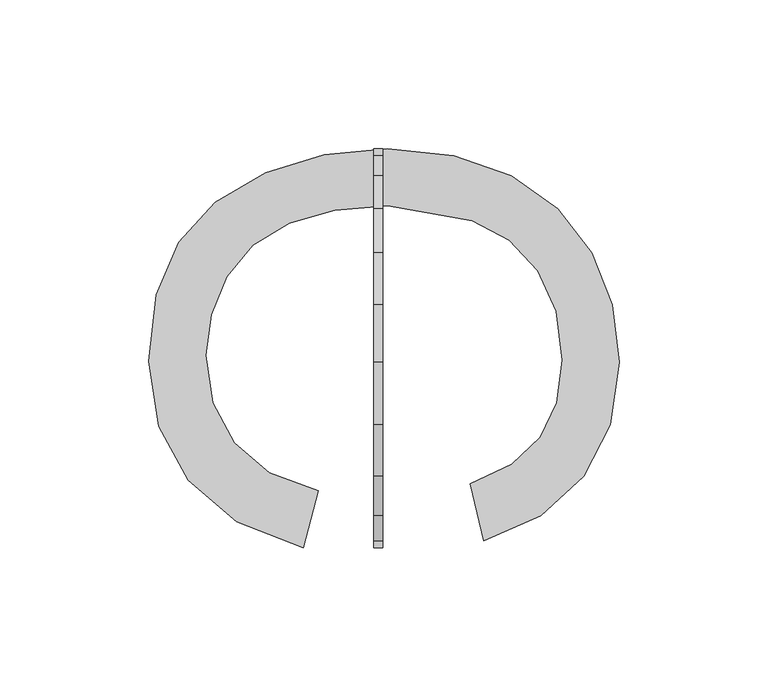
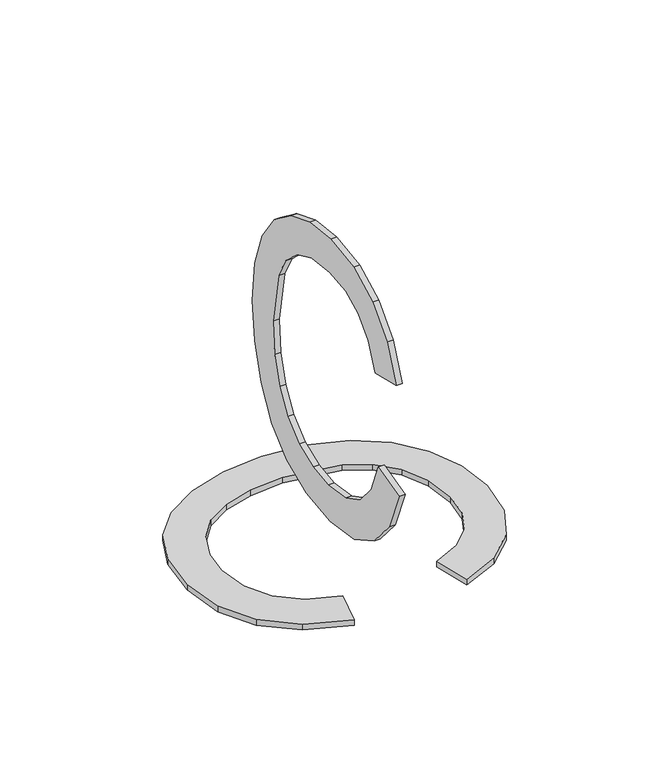
"""IFC4 building model written with IfcOpenShell, lengths in millimetres: proxy geometry, Grid Number2_FedEx : Grid Number2_FedEx."""

import ifcopenshell
import ifcopenshell.guid

model = None  # the IFC model being written
_history = None  # IfcOwnerHistory: only IFC2X3 demands one
_inside = {}  # id of a spatial element -> (the spatial element, [elements in it])
_under = {}  # id of a project, library or spatial element -> (it, [spatial elements below it])
_declared = {}  # id of a project -> (the project, [libraries it declares])
_typed = {}  # id of a type object -> (the type object, [elements of that type])
_made_of = {}  # id of a material, layer set ... -> (it, [elements and type objects made of it])


def new_model(schema):
    """Start an empty IFC model of exactly this schema.

    Asked for "IFC4X3", IfcOpenShell would pick the latest addendum, in which some entities
    have other attributes; the version numbers below select the first issue.
    IFC2X3 requires an IfcOwnerHistory on every rooted entity: one is made here for all.
    """
    global model, _history
    if schema == "IFC4X3":
        model = ifcopenshell.file(schema_version=(4, 3, 0, 0))
    else:
        model = ifcopenshell.file(schema=schema)
    _inside.clear()
    _under.clear()
    _declared.clear()
    _typed.clear()
    _made_of.clear()
    _history = None
    if model.schema == "IFC2X3":
        org = make("IfcOrganization", Name="unknown")
        user = make(
            "IfcPersonAndOrganization",
            ThePerson=make("IfcPerson", FamilyName="unknown"),
            TheOrganization=org,
        )
        app = make(
            "IfcApplication",
            ApplicationDeveloper=org,
            Version="unknown",
            ApplicationFullName="unknown",
            ApplicationIdentifier="unknown",
        )
        _history = make(
            "IfcOwnerHistory",
            OwningUser=user,
            OwningApplication=app,
            ChangeAction="ADDED",
            CreationDate=0,
        )
    return model


def make(cls, **values):
    """One entity of the class cls with the attributes given. An attribute that is None is left unset."""
    return model.create_entity(
        cls, **{name: value for name, value in values.items() if value is not None}
    )


def rooted(cls, **values):
    """An entity with a GlobalId (a new one), such as an element, a storey or a relation."""
    return make(cls, GlobalId=ifcopenshell.guid.new(), OwnerHistory=_history, **values)


def si_unit(unit_type, name, prefix=None):
    """IfcSIUnit, for example si_unit("LENGTHUNIT", "METRE", prefix="MILLI")."""
    return make("IfcSIUnit", UnitType=unit_type, Prefix=prefix, Name=name)


def assignment(units):
    """IfcUnitAssignment: the units of a project."""
    return None if units is None else make("IfcUnitAssignment", Units=units)


def point(xyz):
    """IfcCartesianPoint."""
    return None if xyz is None else make("IfcCartesianPoint", Coordinates=xyz)


def direction(xyz):
    """IfcDirection."""
    return None if xyz is None else make("IfcDirection", DirectionRatios=xyz)


def frame(location, z_axis=None, x_axis=None):
    """IfcAxis2Placement3D, a coordinate frame: its origin and axes. An axis left out is left unset."""
    return make(
        "IfcAxis2Placement3D",
        Location=point(location),
        Axis=direction(z_axis),
        RefDirection=direction(x_axis),
    )


def origin():
    """The frame at (0, 0, 0) with its axes left unset."""
    return frame((0.0, 0.0, 0.0))


def origin_with_axes():
    """The frame at (0, 0, 0) with the z axis (0, 0, 1) and the x axis (1, 0, 0) written out."""
    return frame((0.0, 0.0, 0.0), z_axis=(0.0, 0.0, 1.0), x_axis=(1.0, 0.0, 0.0))


def place(relative_to, where):
    """IfcLocalPlacement: puts the frame where relative to a parent placement (None: the world)."""
    return make(
        "IfcLocalPlacement", PlacementRelTo=relative_to, RelativePlacement=where
    )


def context(
    kind, dimensions, precision=None, world=None, true_north=None, identifier=None
):
    """IfcGeometricRepresentationContext, for example the 3D "Model" context."""
    return make(
        "IfcGeometricRepresentationContext",
        ContextIdentifier=identifier,
        ContextType=kind,
        CoordinateSpaceDimension=dimensions,
        Precision=precision,
        WorldCoordinateSystem=world,
        TrueNorth=true_north,
    )


def project(units=None, contexts=None):
    """IfcProject with its units and contexts."""
    return rooted(
        "IfcProject",
        Name="project",
        RepresentationContexts=contexts,
        UnitsInContext=assignment(units),
    )


def spatial(cls, under=None, at=None, **own):
    """A site, building, storey or space (cls), placed at a placement, below another one or the project."""
    s = rooted(cls, ObjectPlacement=at, **own)
    if under is not None:
        _under.setdefault(under.id(), (under, []))[1].append(s)
    return s


def polyline(points):
    """IfcPolyline through the points."""
    return make("IfcPolyline", Points=[point(p) for p in points])


def outline(outer, holes=None, kind="AREA"):
    """IfcArbitraryClosedProfileDef: a profile drawn as a closed curve; with holes, ...WithVoids."""
    if holes is None:
        return make("IfcArbitraryClosedProfileDef", ProfileType=kind, OuterCurve=outer)
    return make(
        "IfcArbitraryProfileDefWithVoids",
        ProfileType=kind,
        OuterCurve=outer,
        InnerCurves=holes,
    )


def extrude(swept, where, along, depth):
    """IfcExtrudedAreaSolid: the profile swept, set in the frame where, extruded along a direction by depth."""
    return make(
        "IfcExtrudedAreaSolid",
        SweptArea=swept,
        Position=where,
        ExtrudedDirection=direction(along),
        Depth=depth,
    )


def shape(context_of_items, identifier, shape_type, items):
    """IfcShapeRepresentation: the items that make up one representation, for example the "Body"."""
    return make(
        "IfcShapeRepresentation",
        ContextOfItems=context_of_items,
        RepresentationIdentifier=identifier,
        RepresentationType=shape_type,
        Items=items,
    )


def source(mapping_origin, context_of_items, identifier, shape_type, items):
    """IfcRepresentationMap: a shape defined once, which mapped items show again and again."""
    return make(
        "IfcRepresentationMap",
        MappingOrigin=mapping_origin,
        MappedRepresentation=shape(context_of_items, identifier, shape_type, items),
    )


def transform(
    local_origin,
    x_axis=None,
    y_axis=None,
    z_axis=None,
    scale=None,
    scale2=None,
    scale3=None,
    uniform=True,
):
    """IfcCartesianTransformationOperator3D, or its non-uniform kind. x_axis, y_axis, z_axis: its Axis1, 2, 3."""
    if uniform:
        return make(
            "IfcCartesianTransformationOperator3D",
            Axis1=direction(x_axis),
            Axis2=direction(y_axis),
            LocalOrigin=point(local_origin),
            Scale=scale,
            Axis3=direction(z_axis),
        )
    return make(
        "IfcCartesianTransformationOperator3DnonUniform",
        Axis1=direction(x_axis),
        Axis2=direction(y_axis),
        LocalOrigin=point(local_origin),
        Scale=scale,
        Axis3=direction(z_axis),
        Scale2=scale2,
        Scale3=scale3,
    )


def mapped(mapping_source, mapping_target):
    """IfcMappedItem: shows the shape of a source again, moved by a transform."""
    return make(
        "IfcMappedItem", MappingSource=mapping_source, MappingTarget=mapping_target
    )


def made_of(thing, what):
    """Note that an element or type object is made of a material, layer set ...; save() writes the relation."""
    if what is not None:
        _made_of.setdefault(what.id(), (what, []))[1].append(thing)
    return thing


def element(
    cls,
    number,
    at=None,
    inside=None,
    cuts=None,
    type_object=None,
    material=None,
    context=None,
    identifier="Body",
    shape_type=None,
    held_by="IfcProductDefinitionShape",
    body=None,
    shapes=None,
    **own,
):
    """One element of the class cls, such as IfcWall. Its Tag is "e" and its number.

    at: its placement. inside: the storey or other place that contains it. cuts: it is an
    opening in that element (IfcRelVoidsElement). A single representation is given by context,
    identifier, shape_type and body (its items); several are given by shapes. held_by: the class
    of the entity that holds the representations. save() writes the other relations.
    """
    e = rooted(cls, Tag="e%d" % number, ObjectPlacement=at, **own)
    if body is not None:
        shapes = [shape(context, identifier, shape_type, body)]
    if shapes is not None:
        e.Representation = make(held_by, Representations=shapes)
    if inside is not None:
        _inside.setdefault(inside.id(), (inside, []))[1].append(e)
    if cuts is not None:
        rooted(
            "IfcRelVoidsElement", RelatingBuildingElement=cuts, RelatedOpeningElement=e
        )
    if type_object is not None:
        _typed.setdefault(type_object.id(), (type_object, []))[1].append(e)
    return made_of(e, material)


def aggregate(whole, parts):
    """IfcRelAggregates: a whole, such as a stair, and the parts it consists of."""
    return rooted("IfcRelAggregates", RelatingObject=whole, RelatedObjects=parts)


def save(model, path):
    """Write the relations noted so far, then the file.

    IfcRelAggregates (storeys below a building ...), IfcRelContainedInSpatialStructure (elements
    in a storey), IfcRelDefinesByType, IfcRelAssociatesMaterial and IfcRelDeclares: one each for
    every whole, place, type object, material and project.
    """
    for whole, parts in _under.values():
        aggregate(whole, parts)
    for where, things in _inside.values():
        rooted(
            "IfcRelContainedInSpatialStructure",
            RelatedElements=things,
            RelatingStructure=where,
        )
    for kind, things in _typed.values():
        rooted("IfcRelDefinesByType", RelatedObjects=things, RelatingType=kind)
    for what, things in _made_of.values():
        rooted("IfcRelAssociatesMaterial", RelatedObjects=things, RelatingMaterial=what)
    for by, libraries in _declared.values():
        rooted("IfcRelDeclares", RelatingContext=by, RelatedDefinitions=libraries)
    model.write(path)


def entourage_e42254bd(model_context):
    return source(origin(), model_context, "Body", "SweptSolid", [
        extrude(outline(polyline([(-129.8532903, 174.6783588), (-134.7870294, 155.5414317), (-157.086969, 164.3717033), (-173.3785864, 178.2291558), (-183.3441786, 196.4316626), (-186.6660426, 218.2970969), (-184.1524521, 240.4942504), (-176.6116805, 258.1220887), (-164.3053656, 271.6338058), (-147.495145, 281.4825954), (-127.7321563, 287.4955898), (-106.5675373, 289.4999213), (-84.2442371, 287.2339522), (-64.967147, 280.4360447), (-49.3483122, 269.4612787), (-37.999778, 254.6647337), (-31.0897401, 237.1163211), (-28.7863942, 217.885952), (-31.7671948, 196.9035449), (-40.7095968, 179.5560326), (-55.0622921, 166.3853789), (-74.2739728, 157.9335476), (-78.8339437, 177.0704747), (-64.878377, 183.7048586), (-55.3052414, 192.7687352), (-49.7688013, 204.3742349), (-47.9233213, 218.6334882), (-49.9697017, 235.0699407), (-56.1088428, 248.5723136), (-65.6959948, 258.8182318), (-78.0864075, 265.4853204), (-106.5301605, 270.3629942), (-124.2093919, 268.9193149), (-139.4965075, 264.588277), (-151.8074945, 257.2063569), (-160.5583403, 246.610031), (-165.7864217, 233.9065875), (-167.5291155, 220.2033143), (-165.1556881, 204.2293998), (-158.0354056, 190.9185831), (-146.2430218, 180.8688931), (-129.8532903, 174.6783588)])), origin_with_axes(), (0.0, 0.0, 1.0), 3.175),
        extrude(outline(polyline([(174.6783588, 68.6589117), (180.8688931, 52.2691802), (190.9185831, 40.4767964), (204.2293998, 33.356514), (220.2033143, 30.9830865), (233.9065875, 32.7257803), (246.610031, 37.9538617), (257.2063569, 46.7047075), (264.588277, 59.0156945), (268.9193149, 74.3028101), (270.3629942, 91.9820416), (265.4853204, 120.4257945), (258.8182318, 132.8162073), (248.5723136, 142.4033592), (235.0699407, 148.5425004), (218.6334882, 150.5888808), (204.3742349, 148.7434007), (192.7687352, 143.2069607), (183.7048586, 133.633825), (177.0704747, 119.6782583), (157.9335476, 124.2382292), (166.3853789, 143.4499099), (179.5560326, 157.8026052), (196.9035449, 166.7450072), (217.885952, 169.7258079), (237.1163211, 167.4224619), (254.6647337, 160.512424), (269.4612787, 149.1638899), (280.4360447, 133.5450551), (287.2339522, 114.267965), (289.4999213, 91.9446648), (287.4955898, 70.7800457), (281.4825954, 51.017057), (271.6338058, 34.2068364), (258.1220887, 21.9005215), (240.4942504, 14.3597499), (218.2970969, 11.8461594), (196.4316626, 15.1680235), (178.2291558, 25.1336156), (164.3717033, 41.425233), (155.5414317, 63.7251727), (174.6783588, 68.6589117)])), frame((-111.2489267, 0.0, 0.0), z_axis=(1.0, 0.0, 0.0), x_axis=(0.0, 1.0, 0.0)), (0.0, 0.0, 1.0), 3.175),
    ])


if __name__ == "__main__":
    model = new_model("IFC4")
    model_context = context("Model", 3, world=origin())
    ifc_project = project(units=[si_unit("LENGTHUNIT", "METRE", prefix="MILLI")], contexts=[model_context])
    site = spatial("IfcSite", under=ifc_project)
    building = spatial("IfcBuilding", under=site)
    placement = place(None, origin())
    entourage_shape = entourage_e42254bd(model_context)
    element("IfcBuildingElementProxy", 1, Name="Grid Number2_FedEx : Grid Number2_FedEx", ObjectType="Grid Number2_FedEx : Grid Number2_FedEx", at=placement, inside=building, context=model_context, shape_type="MappedRepresentation", body=[
        mapped(entourage_shape, transform((0.0, 0.0, 0.0), x_axis=(1.0, 0.0, 0.0), y_axis=(0.0, 1.0, 0.0), z_axis=(0.0, 0.0, 1.0))),
    ])
    save(model, "model.ifc")

# Revit data of these elements
# Type "Grid Number2_FedEx : Grid Number2_FedEx"
#   Grid [instance default] = "S"
#   Label Width [instance default] = 1' - 0"
#   Half Box Width2 [instance default] = 0' - 6.13846"
#   Half Box Width [instance default] = 0' - 6"
#   Robust [instance default] = yes
#   Height = 0
#   Assembly Code = ""
# Element 1 (IfcBuildingElementProxy, "Grid Number2_FedEx : Grid Number2_FedEx")
#   Grid = "C"
#   Robust = no
#   Materials on its faces: "Letter"
# Materials
#   "Letter": class "Unassigned", colour RGB 178 187 30, transparency 0, Comments = "Rendering appearance not upgraded "
